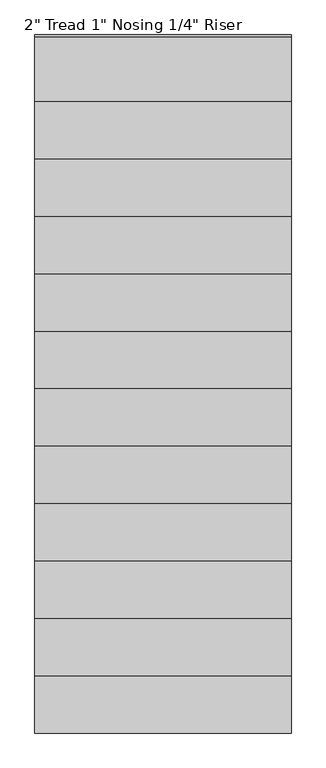
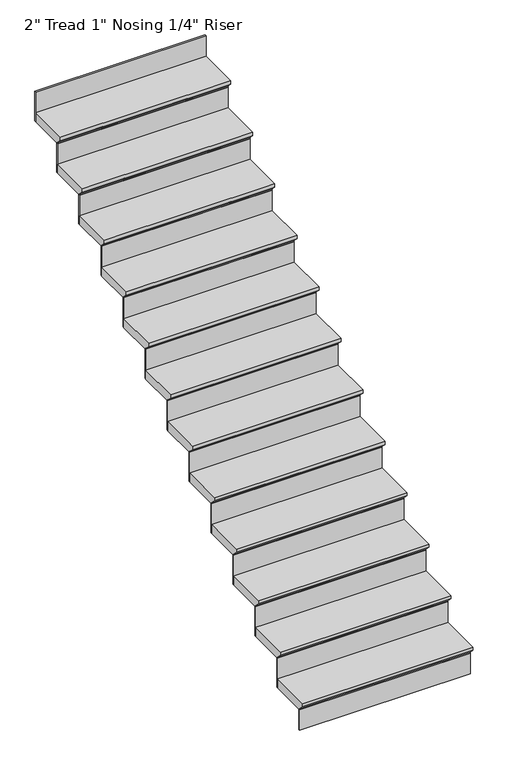
"""IFC4 building model written with IfcOpenShell, lengths in millimetres: stair flight geometry."""

from ifc_helpers import new_model, si_unit, frame, origin, place, context, project, spatial, polyline, outline, extrude, source, transform, mapped, element, save


def stair_flight_5e37eb87(model_context):
    return source(origin(), model_context, "Body", "SweptSolid", [
        extrude(outline(polyline([(-12572.2570712, -1998.7846154), (-12343.6570712, -1998.7846154), (-12343.6570712, -2049.5846154), (-12546.8570712, -2049.5846154), (-12546.8570712, -2043.2346154), (-12572.2570712, -2017.8346154), (-12572.2570712, -1998.7846154)])), frame((-25042.4664763, 0.0, 0.0), z_axis=(1.0, 0.0, 0.0), x_axis=(0.0, 1.0, 0.0)), (0.0, 0.0, 1.0), 908.05),
        extrude(outline(polyline([(-24134.4164763, -12540.5070712), (-24134.4164763, -12546.8570712), (-25042.4664763, -12546.8570712), (-25042.4664763, -12540.5070712), (-24134.4164763, -12540.5070712)])), frame((0.0, 0.0, -2165.35), z_axis=(0.0, 0.0, 1.0), x_axis=(1.0, 0.0, 0.0)), (0.0, 0.0, 1.0), 115.7653846),
        extrude(outline(polyline([(-24134.4164763, -12337.3070712), (-24134.4164763, -12343.6570712), (-25042.4664763, -12343.6570712), (-25042.4664763, -12337.3070712), (-24134.4164763, -12337.3070712)])), frame((0.0, 0.0, -2049.5846154), z_axis=(0.0, 0.0, 1.0), x_axis=(1.0, 0.0, 0.0)), (0.0, 0.0, 1.0), 166.5653846),
        extrude(outline(polyline([(-12369.0570712, -1832.2192308), (-12140.4570712, -1832.2192308), (-12140.4570712, -1883.0192308), (-12343.6570712, -1883.0192308), (-12343.6570712, -1876.6692308), (-12369.0570712, -1851.2692308), (-12369.0570712, -1832.2192308)])), frame((-25042.4664763, 0.0, 0.0), z_axis=(1.0, 0.0, 0.0), x_axis=(0.0, 1.0, 0.0)), (0.0, 0.0, 1.0), 908.05),
        extrude(outline(polyline([(-24134.4164763, -12134.1070712), (-24134.4164763, -12140.4570712), (-25042.4664763, -12140.4570712), (-25042.4664763, -12134.1070712), (-24134.4164763, -12134.1070712)])), frame((0.0, 0.0, -1883.0192308), z_axis=(0.0, 0.0, 1.0), x_axis=(1.0, 0.0, 0.0)), (0.0, 0.0, 1.0), 166.5653846),
        extrude(outline(polyline([(-12165.8570712, -1665.6538462), (-11937.2570712, -1665.6538462), (-11937.2570712, -1716.4538462), (-12140.4570712, -1716.4538462), (-12140.4570712, -1710.1038462), (-12165.8570712, -1684.7038462), (-12165.8570712, -1665.6538462)])), frame((-25042.4664763, 0.0, 0.0), z_axis=(1.0, 0.0, 0.0), x_axis=(0.0, 1.0, 0.0)), (0.0, 0.0, 1.0), 908.05),
        extrude(outline(polyline([(-24134.4164763, -11930.9070712), (-24134.4164763, -11937.2570712), (-25042.4664763, -11937.2570712), (-25042.4664763, -11930.9070712), (-24134.4164763, -11930.9070712)])), frame((0.0, 0.0, -1716.4538462), z_axis=(0.0, 0.0, 1.0), x_axis=(1.0, 0.0, 0.0)), (0.0, 0.0, 1.0), 166.5653846),
        extrude(outline(polyline([(-11962.6570712, -1499.0884615), (-11734.0570712, -1499.0884615), (-11734.0570712, -1549.8884615), (-11937.2570712, -1549.8884615), (-11937.2570712, -1543.5384615), (-11962.6570712, -1518.1384615), (-11962.6570712, -1499.0884615)])), frame((-25042.4664763, 0.0, 0.0), z_axis=(1.0, 0.0, 0.0), x_axis=(0.0, 1.0, 0.0)), (0.0, 0.0, 1.0), 908.05),
        extrude(outline(polyline([(-24134.4164763, -11727.7070712), (-24134.4164763, -11734.0570712), (-25042.4664763, -11734.0570712), (-25042.4664763, -11727.7070712), (-24134.4164763, -11727.7070712)])), frame((0.0, 0.0, -1549.8884615), z_axis=(0.0, 0.0, 1.0), x_axis=(1.0, 0.0, 0.0)), (0.0, 0.0, 1.0), 166.5653846),
        extrude(outline(polyline([(-11759.4570712, -1332.5230769), (-11530.8570712, -1332.5230769), (-11530.8570712, -1383.3230769), (-11734.0570712, -1383.3230769), (-11734.0570712, -1376.9730769), (-11759.4570712, -1351.5730769), (-11759.4570712, -1332.5230769)])), frame((-25042.4664763, 0.0, 0.0), z_axis=(1.0, 0.0, 0.0), x_axis=(0.0, 1.0, 0.0)), (0.0, 0.0, 1.0), 908.05),
        extrude(outline(polyline([(-24134.4164763, -11524.5070712), (-24134.4164763, -11530.8570712), (-25042.4664763, -11530.8570712), (-25042.4664763, -11524.5070712), (-24134.4164763, -11524.5070712)])), frame((0.0, 0.0, -1383.3230769), z_axis=(0.0, 0.0, 1.0), x_axis=(1.0, 0.0, 0.0)), (0.0, 0.0, 1.0), 166.5653846),
        extrude(outline(polyline([(-11556.2570712, -1165.9576923), (-11327.6570712, -1165.9576923), (-11327.6570712, -1216.7576923), (-11530.8570712, -1216.7576923), (-11530.8570712, -1210.4076923), (-11556.2570712, -1185.0076923), (-11556.2570712, -1165.9576923)])), frame((-25042.4664763, 0.0, 0.0), z_axis=(1.0, 0.0, 0.0), x_axis=(0.0, 1.0, 0.0)), (0.0, 0.0, 1.0), 908.05),
        extrude(outline(polyline([(-24134.4164763, -11321.3070712), (-24134.4164763, -11327.6570712), (-25042.4664763, -11327.6570712), (-25042.4664763, -11321.3070712), (-24134.4164763, -11321.3070712)])), frame((0.0, 0.0, -1216.7576923), z_axis=(0.0, 0.0, 1.0), x_axis=(1.0, 0.0, 0.0)), (0.0, 0.0, 1.0), 166.5653846),
        extrude(outline(polyline([(-11353.0570712, -999.3923077), (-11124.4570712, -999.3923077), (-11124.4570712, -1050.1923077), (-11327.6570712, -1050.1923077), (-11327.6570712, -1043.8423077), (-11353.0570712, -1018.4423077), (-11353.0570712, -999.3923077)])), frame((-25042.4664763, 0.0, 0.0), z_axis=(1.0, 0.0, 0.0), x_axis=(0.0, 1.0, 0.0)), (0.0, 0.0, 1.0), 908.05),
        extrude(outline(polyline([(-24134.4164763, -11118.1070712), (-24134.4164763, -11124.4570712), (-25042.4664763, -11124.4570712), (-25042.4664763, -11118.1070712), (-24134.4164763, -11118.1070712)])), frame((0.0, 0.0, -1050.1923077), z_axis=(0.0, 0.0, 1.0), x_axis=(1.0, 0.0, 0.0)), (0.0, 0.0, 1.0), 166.5653846),
        extrude(outline(polyline([(-11149.8570712, -832.8269231), (-10921.2570712, -832.8269231), (-10921.2570712, -883.6269231), (-11124.4570712, -883.6269231), (-11124.4570712, -877.2769231), (-11149.8570712, -851.8769231), (-11149.8570712, -832.8269231)])), frame((-25042.4664763, 0.0, 0.0), z_axis=(1.0, 0.0, 0.0), x_axis=(0.0, 1.0, 0.0)), (0.0, 0.0, 1.0), 908.05),
        extrude(outline(polyline([(-24134.4164763, -10914.9070712), (-24134.4164763, -10921.2570712), (-25042.4664763, -10921.2570712), (-25042.4664763, -10914.9070712), (-24134.4164763, -10914.9070712)])), frame((0.0, 0.0, -883.6269231), z_axis=(0.0, 0.0, 1.0), x_axis=(1.0, 0.0, 0.0)), (0.0, 0.0, 1.0), 166.5653846),
        extrude(outline(polyline([(-10946.6570712, -666.2615385), (-10718.0570712, -666.2615385), (-10718.0570712, -717.0615385), (-10921.2570712, -717.0615385), (-10921.2570712, -710.7115385), (-10946.6570712, -685.3115385), (-10946.6570712, -666.2615385)])), frame((-25042.4664763, 0.0, 0.0), z_axis=(1.0, 0.0, 0.0), x_axis=(0.0, 1.0, 0.0)), (0.0, 0.0, 1.0), 908.05),
        extrude(outline(polyline([(-24134.4164763, -10711.7070712), (-24134.4164763, -10718.0570712), (-25042.4664763, -10718.0570712), (-25042.4664763, -10711.7070712), (-24134.4164763, -10711.7070712)])), frame((0.0, 0.0, -717.0615385), z_axis=(0.0, 0.0, 1.0), x_axis=(1.0, 0.0, 0.0)), (0.0, 0.0, 1.0), 166.5653846),
        extrude(outline(polyline([(-10743.4570712, -499.6961538), (-10514.8570712, -499.6961538), (-10514.8570712, -550.4961538), (-10718.0570712, -550.4961538), (-10718.0570712, -544.1461538), (-10743.4570712, -518.7461538), (-10743.4570712, -499.6961538)])), frame((-25042.4664763, 0.0, 0.0), z_axis=(1.0, 0.0, 0.0), x_axis=(0.0, 1.0, 0.0)), (0.0, 0.0, 1.0), 908.05),
        extrude(outline(polyline([(-24134.4164763, -10508.5070712), (-24134.4164763, -10514.8570712), (-25042.4664763, -10514.8570712), (-25042.4664763, -10508.5070712), (-24134.4164763, -10508.5070712)])), frame((0.0, 0.0, -550.4961538), z_axis=(0.0, 0.0, 1.0), x_axis=(1.0, 0.0, 0.0)), (0.0, 0.0, 1.0), 166.5653846),
        extrude(outline(polyline([(-10540.2570712, -333.1307692), (-10311.6570712, -333.1307692), (-10311.6570712, -383.9307692), (-10514.8570712, -383.9307692), (-10514.8570712, -377.5807692), (-10540.2570712, -352.1807692), (-10540.2570712, -333.1307692)])), frame((-25042.4664763, 0.0, 0.0), z_axis=(1.0, 0.0, 0.0), x_axis=(0.0, 1.0, 0.0)), (0.0, 0.0, 1.0), 908.05),
        extrude(outline(polyline([(-24134.4164763, -10305.3070712), (-24134.4164763, -10311.6570712), (-25042.4664763, -10311.6570712), (-25042.4664763, -10305.3070712), (-24134.4164763, -10305.3070712)])), frame((0.0, 0.0, -383.9307692), z_axis=(0.0, 0.0, 1.0), x_axis=(1.0, 0.0, 0.0)), (0.0, 0.0, 1.0), 166.5653846),
        extrude(outline(polyline([(-24134.4164763, -10102.1070712), (-24134.4164763, -10108.4570712), (-25042.4664763, -10108.4570712), (-25042.4664763, -10102.1070712), (-24134.4164763, -10102.1070712)])), frame((0.0, 0.0, -217.3653846), z_axis=(0.0, 0.0, 1.0), x_axis=(1.0, 0.0, 0.0)), (0.0, 0.0, 1.0), 166.5653846),
        extrude(outline(polyline([(-10337.0570712, -166.5653846), (-10108.4570712, -166.5653846), (-10108.4570712, -217.3653846), (-10311.6570712, -217.3653846), (-10311.6570712, -211.0153846), (-10337.0570712, -185.6153846), (-10337.0570712, -166.5653846)])), frame((-25042.4664763, 0.0, 0.0), z_axis=(1.0, 0.0, 0.0), x_axis=(0.0, 1.0, 0.0)), (0.0, 0.0, 1.0), 908.05),
    ])


if __name__ == "__main__":
    model = new_model("IFC4")
    model_context = context("Model", 3, world=origin())
    ifc_project = project(units=[si_unit("LENGTHUNIT", "METRE", prefix="MILLI")], contexts=[model_context])
    site = spatial("IfcSite", under=ifc_project)
    building = spatial("IfcBuilding", under=site)
    placement = place(None, origin())
    stair_flight_shape = stair_flight_5e37eb87(model_context)
    element("IfcStairFlight", 1, ObjectType="2\" Tread 1\" Nosing 1/4\" Riser", at=placement, inside=building, context=model_context, shape_type="MappedRepresentation", body=[
        mapped(stair_flight_shape, transform((0.0, 0.0, 0.0), x_axis=(1.0, 0.0, 0.0), y_axis=(0.0, 1.0, 0.0), z_axis=(0.0, 0.0, 1.0))),
    ])
    save(model, "model.ifc")
